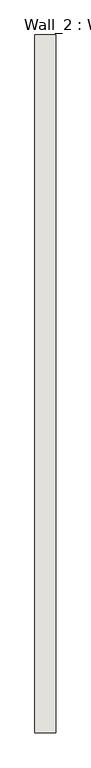
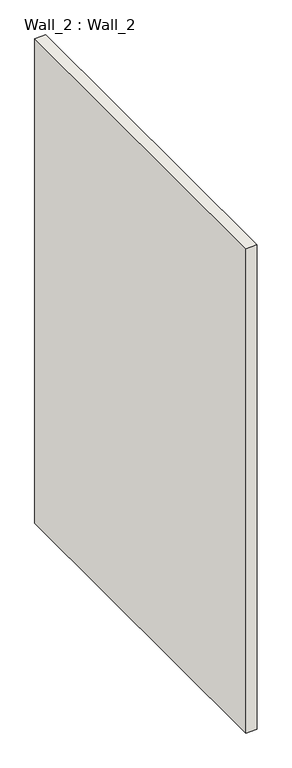
"""IFC4 building model written with IfcOpenShell, lengths in millimetres: wall geometry, Wall_2 : Wall_2."""

from ifc_helpers import new_model, si_unit, origin, origin_with_axes, place, context, project, spatial, polyline, outline, extrude, source, transform, mapped, element, save


def wall_2_wall_2_345a8b54(model_context):
    return source(origin(), model_context, "Body", "SweptSolid", [
        extrude(outline(polyline([(100.0, 7510.0), (100.0, 4150.0), (0.0, 4150.0), (0.0, 7510.0), (100.0, 7510.0)])), origin_with_axes(), (0.0, 0.0, 1.0), 4700.0),
    ])


if __name__ == "__main__":
    model = new_model("IFC4")
    model_context = context("Model", 3, world=origin())
    ifc_project = project(units=[si_unit("LENGTHUNIT", "METRE", prefix="MILLI")], contexts=[model_context])
    site = spatial("IfcSite", under=ifc_project)
    building = spatial("IfcBuilding", under=site)
    placement = place(None, origin())
    wall_2_wall_2_shape = wall_2_wall_2_345a8b54(model_context)
    element("IfcWall", 1, ObjectType="Wall_2 : Wall_2", at=placement, inside=building, context=model_context, shape_type="MappedRepresentation", body=[
        mapped(wall_2_wall_2_shape, transform((0.0, 0.0, 0.0), x_axis=(1.0, 0.0, 0.0), y_axis=(0.0, 1.0, 0.0), z_axis=(0.0, 0.0, 1.0))),
    ])
    save(model, "model.ifc")

# Revit data of these elements
# Type "Wall_2 : Wall_2"
#   NameOverride = "Wall_2"
# Element 1 (IfcWall, "Wall_2 : Wall_2")
#   Materials on its faces: "IfcSurfaceStyle #33"
# Materials
#   "IfcSurfaceStyle #33": class "Unassigned", colour RGB 214 214 214, transparency 0
